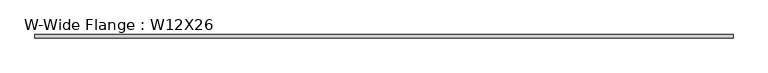
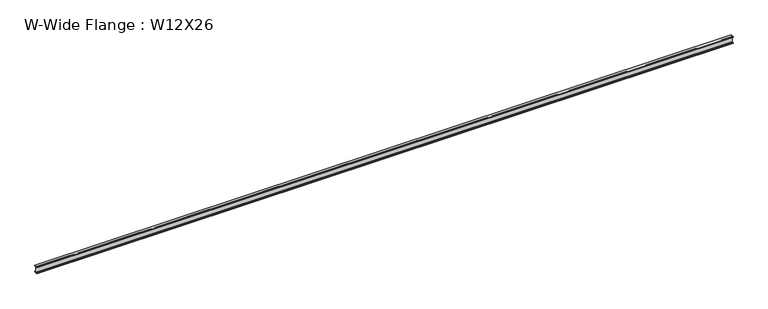
"""IFC4 building model written with IfcOpenShell, lengths in millimetres: beam geometry, W-Wide Flange : W12X26."""

from ifc_helpers import new_model, si_unit, point, frame, frame_2d, origin, place, context, project, spatial, polyline, circle_curve, trimmed, segment, composite_curve, outline, extrude, source, transform, mapped, element, save


def w_wide_flange_w12x26_a4173b93(model_context):
    return source(origin(), model_context, "Body", "SweptSolid", [
        extrude(outline(composite_curve([segment(polyline([(82.4011719, -145.5539063), (82.4011719, -155.178125), (-82.4011719, -155.178125), (-82.4011719, -145.5539063), (-20.2902344, -145.5539063)]), True, "CONTINUOUS"), segment(trimmed(circle_curve(frame_2d((-20.2902344, -128.190625)), 17.3632812), [point((-20.2902344, -145.5539063))], [point((-2.9269531, -128.190625))], True, "CARTESIAN"), True, "CONTINUOUS"), segment(polyline([(-2.9269531, -128.190625), (-2.9269531, 128.190625)]), True, "CONTINUOUS"), segment(trimmed(circle_curve(frame_2d((-20.2902344, 128.190625)), 17.3632812), [point((-2.9269531, 128.190625))], [point((-20.2902344, 145.5539062))], True, "CARTESIAN"), True, "CONTINUOUS"), segment(polyline([(-20.2902344, 145.5539062), (-82.4011719, 145.5539062), (-82.4011719, 155.178125), (82.4011719, 155.178125), (82.4011719, 145.5539062), (20.2902344, 145.5539062)]), True, "CONTINUOUS"), segment(trimmed(circle_curve(frame_2d((20.2902344, 128.190625)), 17.3632812), [point((20.2902344, 145.5539062))], [point((2.9269531, 128.190625))], True, "CARTESIAN"), True, "CONTINUOUS"), segment(polyline([(2.9269531, 128.190625), (2.9269531, -128.190625)]), True, "CONTINUOUS"), segment(trimmed(circle_curve(frame_2d((20.2902344, -128.190625)), 17.3632812), [point((2.9269531, -128.190625))], [point((20.2902344, -145.5539063))], True, "CARTESIAN"), True, "CONTINUOUS"), segment(polyline([(20.2902344, -145.5539063), (82.4011719, -145.5539063)]), True, "CONTINUOUS")], self_intersect=False)), frame((-30805.35213, 0.0, 0.0), z_axis=(1.0, 0.0, 0.0), x_axis=(0.0, 1.0, 0.0)), (0.0, 0.0, 1.0), 32919.7151756),
    ])


if __name__ == "__main__":
    model = new_model("IFC4")
    model_context = context("Model", 3, world=origin())
    ifc_project = project(units=[si_unit("LENGTHUNIT", "METRE", prefix="MILLI")], contexts=[model_context])
    site = spatial("IfcSite", under=ifc_project)
    building = spatial("IfcBuilding", under=site)
    placement = place(None, origin())
    w_wide_flange_w12x26_shape = w_wide_flange_w12x26_a4173b93(model_context)
    element("IfcBeam", 1, ObjectType="W-Wide Flange : W12X26", at=placement, inside=building, context=model_context, shape_type="MappedRepresentation", body=[
        mapped(w_wide_flange_w12x26_shape, transform((0.0, 0.0, 0.0), x_axis=(1.0, 0.0, 0.0), y_axis=(0.0, 1.0, 0.0), z_axis=(0.0, 0.0, 1.0))),
    ])
    save(model, "model.ifc")

# Revit data of these elements
# Type "W-Wide Flange : W12X26"
#   Assembly Code = "B10"
#   W = 26
#   Length [instance default] = 5' - 0"
#   bf = 0' - 6 125/256"
#   d = 1' - 0 7/32"
#   k = 0' - 1 1/16"
#   k2 = 0' - 0 175/256"
#   tf = 0' - 0 97/256"
#   tw = 0' - 0 59/256"
#   A = 0.053125 SF
#   Structural Material [instance default] = none
